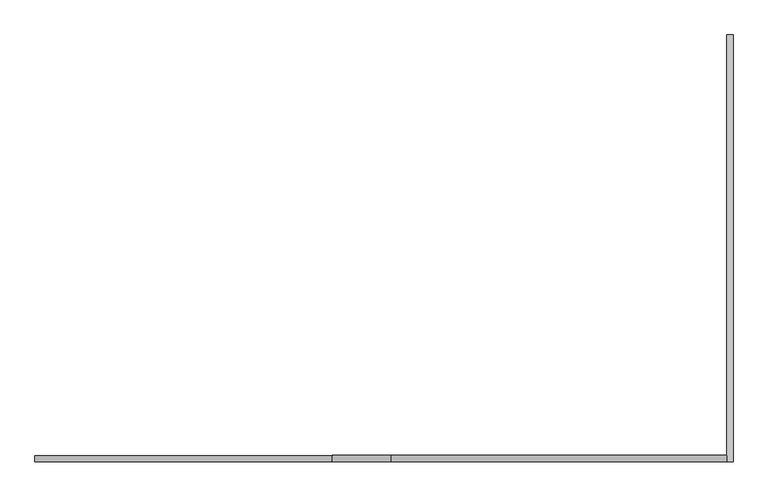
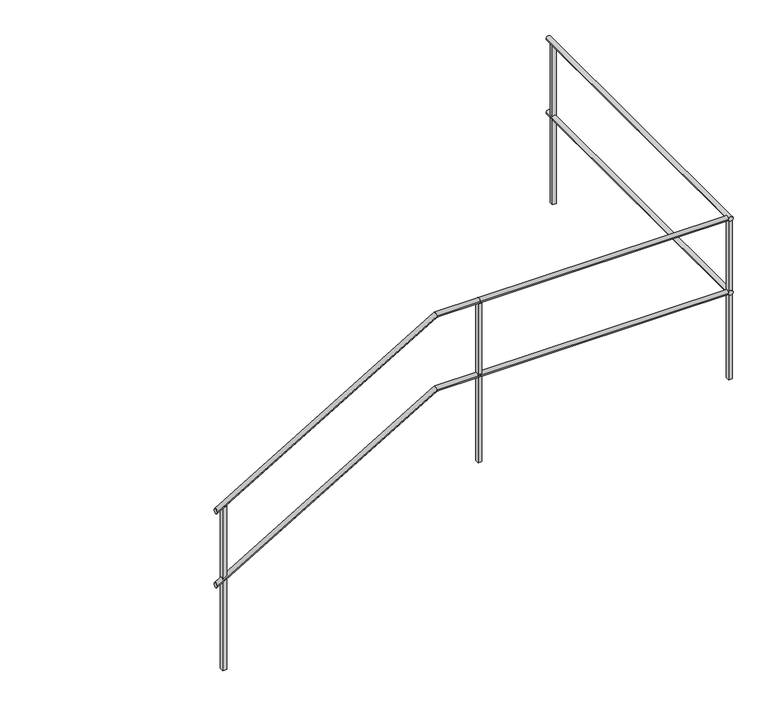
"""IFC4 building model written with IfcOpenShell, lengths in millimetres: railing geometry."""

import ifcopenshell
import ifcopenshell.guid

model = None  # the IFC model being written
_history = None  # IfcOwnerHistory: only IFC2X3 demands one
_inside = {}  # id of a spatial element -> (the spatial element, [elements in it])
_under = {}  # id of a project, library or spatial element -> (it, [spatial elements below it])
_declared = {}  # id of a project -> (the project, [libraries it declares])
_typed = {}  # id of a type object -> (the type object, [elements of that type])
_made_of = {}  # id of a material, layer set ... -> (it, [elements and type objects made of it])


def new_model(schema):
    """Start an empty IFC model of exactly this schema.

    Asked for "IFC4X3", IfcOpenShell would pick the latest addendum, in which some entities
    have other attributes; the version numbers below select the first issue.
    IFC2X3 requires an IfcOwnerHistory on every rooted entity: one is made here for all.
    """
    global model, _history
    if schema == "IFC4X3":
        model = ifcopenshell.file(schema_version=(4, 3, 0, 0))
    else:
        model = ifcopenshell.file(schema=schema)
    _inside.clear()
    _under.clear()
    _declared.clear()
    _typed.clear()
    _made_of.clear()
    _history = None
    if model.schema == "IFC2X3":
        org = make("IfcOrganization", Name="unknown")
        user = make(
            "IfcPersonAndOrganization",
            ThePerson=make("IfcPerson", FamilyName="unknown"),
            TheOrganization=org,
        )
        app = make(
            "IfcApplication",
            ApplicationDeveloper=org,
            Version="unknown",
            ApplicationFullName="unknown",
            ApplicationIdentifier="unknown",
        )
        _history = make(
            "IfcOwnerHistory",
            OwningUser=user,
            OwningApplication=app,
            ChangeAction="ADDED",
            CreationDate=0,
        )
    return model


def make(cls, **values):
    """One entity of the class cls with the attributes given. An attribute that is None is left unset."""
    return model.create_entity(
        cls, **{name: value for name, value in values.items() if value is not None}
    )


def rooted(cls, **values):
    """An entity with a GlobalId (a new one), such as an element, a storey or a relation."""
    return make(cls, GlobalId=ifcopenshell.guid.new(), OwnerHistory=_history, **values)


def si_unit(unit_type, name, prefix=None):
    """IfcSIUnit, for example si_unit("LENGTHUNIT", "METRE", prefix="MILLI")."""
    return make("IfcSIUnit", UnitType=unit_type, Prefix=prefix, Name=name)


def assignment(units):
    """IfcUnitAssignment: the units of a project."""
    return None if units is None else make("IfcUnitAssignment", Units=units)


def point(xyz):
    """IfcCartesianPoint."""
    return None if xyz is None else make("IfcCartesianPoint", Coordinates=xyz)


def direction(xyz):
    """IfcDirection."""
    return None if xyz is None else make("IfcDirection", DirectionRatios=xyz)


def frame(location, z_axis=None, x_axis=None):
    """IfcAxis2Placement3D, a coordinate frame: its origin and axes. An axis left out is left unset."""
    return make(
        "IfcAxis2Placement3D",
        Location=point(location),
        Axis=direction(z_axis),
        RefDirection=direction(x_axis),
    )


def origin():
    """The frame at (0, 0, 0) with its axes left unset."""
    return frame((0.0, 0.0, 0.0))


def place(relative_to, where):
    """IfcLocalPlacement: puts the frame where relative to a parent placement (None: the world)."""
    return make(
        "IfcLocalPlacement", PlacementRelTo=relative_to, RelativePlacement=where
    )


def context(
    kind, dimensions, precision=None, world=None, true_north=None, identifier=None
):
    """IfcGeometricRepresentationContext, for example the 3D "Model" context."""
    return make(
        "IfcGeometricRepresentationContext",
        ContextIdentifier=identifier,
        ContextType=kind,
        CoordinateSpaceDimension=dimensions,
        Precision=precision,
        WorldCoordinateSystem=world,
        TrueNorth=true_north,
    )


def project(units=None, contexts=None):
    """IfcProject with its units and contexts."""
    return rooted(
        "IfcProject",
        Name="project",
        RepresentationContexts=contexts,
        UnitsInContext=assignment(units),
    )


def spatial(cls, under=None, at=None, **own):
    """A site, building, storey or space (cls), placed at a placement, below another one or the project."""
    s = rooted(cls, ObjectPlacement=at, **own)
    if under is not None:
        _under.setdefault(under.id(), (under, []))[1].append(s)
    return s


def polyline(points):
    """IfcPolyline through the points."""
    return make("IfcPolyline", Points=[point(p) for p in points])


def circle_curve(where, radius):
    """IfcCircle in the frame where."""
    return make("IfcCircle", Position=where, Radius=radius)


def ellipse_curve(where, semi_axis1, semi_axis2):
    """IfcEllipse in the frame where."""
    return make(
        "IfcEllipse", Position=where, SemiAxis1=semi_axis1, SemiAxis2=semi_axis2
    )


def outline(outer, holes=None, kind="AREA"):
    """IfcArbitraryClosedProfileDef: a profile drawn as a closed curve; with holes, ...WithVoids."""
    if holes is None:
        return make("IfcArbitraryClosedProfileDef", ProfileType=kind, OuterCurve=outer)
    return make(
        "IfcArbitraryProfileDefWithVoids",
        ProfileType=kind,
        OuterCurve=outer,
        InnerCurves=holes,
    )


def extrude(swept, where, along, depth):
    """IfcExtrudedAreaSolid: the profile swept, set in the frame where, extruded along a direction by depth."""
    return make(
        "IfcExtrudedAreaSolid",
        SweptArea=swept,
        Position=where,
        ExtrudedDirection=direction(along),
        Depth=depth,
    )


def shape(context_of_items, identifier, shape_type, items):
    """IfcShapeRepresentation: the items that make up one representation, for example the "Body"."""
    return make(
        "IfcShapeRepresentation",
        ContextOfItems=context_of_items,
        RepresentationIdentifier=identifier,
        RepresentationType=shape_type,
        Items=items,
    )


def source(mapping_origin, context_of_items, identifier, shape_type, items):
    """IfcRepresentationMap: a shape defined once, which mapped items show again and again."""
    return make(
        "IfcRepresentationMap",
        MappingOrigin=mapping_origin,
        MappedRepresentation=shape(context_of_items, identifier, shape_type, items),
    )


def transform(
    local_origin,
    x_axis=None,
    y_axis=None,
    z_axis=None,
    scale=None,
    scale2=None,
    scale3=None,
    uniform=True,
):
    """IfcCartesianTransformationOperator3D, or its non-uniform kind. x_axis, y_axis, z_axis: its Axis1, 2, 3."""
    if uniform:
        return make(
            "IfcCartesianTransformationOperator3D",
            Axis1=direction(x_axis),
            Axis2=direction(y_axis),
            LocalOrigin=point(local_origin),
            Scale=scale,
            Axis3=direction(z_axis),
        )
    return make(
        "IfcCartesianTransformationOperator3DnonUniform",
        Axis1=direction(x_axis),
        Axis2=direction(y_axis),
        LocalOrigin=point(local_origin),
        Scale=scale,
        Axis3=direction(z_axis),
        Scale2=scale2,
        Scale3=scale3,
    )


def mapped(mapping_source, mapping_target):
    """IfcMappedItem: shows the shape of a source again, moved by a transform."""
    return make(
        "IfcMappedItem", MappingSource=mapping_source, MappingTarget=mapping_target
    )


def made_of(thing, what):
    """Note that an element or type object is made of a material, layer set ...; save() writes the relation."""
    if what is not None:
        _made_of.setdefault(what.id(), (what, []))[1].append(thing)
    return thing


def element(
    cls,
    number,
    at=None,
    inside=None,
    cuts=None,
    type_object=None,
    material=None,
    context=None,
    identifier="Body",
    shape_type=None,
    held_by="IfcProductDefinitionShape",
    body=None,
    shapes=None,
    **own,
):
    """One element of the class cls, such as IfcWall. Its Tag is "e" and its number.

    at: its placement. inside: the storey or other place that contains it. cuts: it is an
    opening in that element (IfcRelVoidsElement). A single representation is given by context,
    identifier, shape_type and body (its items); several are given by shapes. held_by: the class
    of the entity that holds the representations. save() writes the other relations.
    """
    e = rooted(cls, Tag="e%d" % number, ObjectPlacement=at, **own)
    if body is not None:
        shapes = [shape(context, identifier, shape_type, body)]
    if shapes is not None:
        e.Representation = make(held_by, Representations=shapes)
    if inside is not None:
        _inside.setdefault(inside.id(), (inside, []))[1].append(e)
    if cuts is not None:
        rooted(
            "IfcRelVoidsElement", RelatingBuildingElement=cuts, RelatedOpeningElement=e
        )
    if type_object is not None:
        _typed.setdefault(type_object.id(), (type_object, []))[1].append(e)
    return made_of(e, material)


def aggregate(whole, parts):
    """IfcRelAggregates: a whole, such as a stair, and the parts it consists of."""
    return rooted("IfcRelAggregates", RelatingObject=whole, RelatedObjects=parts)


def save(model, path):
    """Write the relations noted so far, then the file.

    IfcRelAggregates (storeys below a building ...), IfcRelContainedInSpatialStructure (elements
    in a storey), IfcRelDefinesByType, IfcRelAssociatesMaterial and IfcRelDeclares: one each for
    every whole, place, type object, material and project.
    """
    for whole, parts in _under.values():
        aggregate(whole, parts)
    for where, things in _inside.values():
        rooted(
            "IfcRelContainedInSpatialStructure",
            RelatedElements=things,
            RelatingStructure=where,
        )
    for kind, things in _typed.values():
        rooted("IfcRelDefinesByType", RelatedObjects=things, RelatingType=kind)
    for what, things in _made_of.values():
        rooted("IfcRelAssociatesMaterial", RelatedObjects=things, RelatingMaterial=what)
    for by, libraries in _declared.values():
        rooted("IfcRelDeclares", RelatingContext=by, RelatedDefinitions=libraries)
    model.write(path)


def plane_surface(at):
    """IfcPlane: the flat surface through the origin of the frame at, square to its z axis."""
    return make("IfcPlane", Position=at)


def cylinder_surface(at, radius):
    """IfcCylindricalSurface: all points at the distance radius from the z axis of the frame at."""
    return make("IfcCylindricalSurface", Position=at, Radius=radius)


def advanced_brep(points, edges, surfaces, faces):
    """IfcAdvancedBrep: a solid bounded by faces that lie on surfaces and meet in shared edges.

    An edge is (start, end): straight between two places in points (the first is 0);
    or (start, end, curve); or (start, end, curve, False) where it runs against its curve.
    A face is (place in surfaces, loops), or (place, loops, False) where it looks against
    its surface's normal. A loop lists edges by number (the first is 1), with a minus sign
    where the edge is run from its end to its start. The first loop is the outer one.
    """
    corners = [point(p) for p in points]
    vertices = [make("IfcVertexPoint", VertexGeometry=c) for c in corners]
    made = []
    for start, end, *more in edges:
        made.append(
            make(
                "IfcEdgeCurve",
                EdgeStart=vertices[start],
                EdgeEnd=vertices[end],
                EdgeGeometry=more[0] if more else make("IfcPolyline", Points=[corners[start], corners[end]]),
                SameSense=more[1] if len(more) > 1 else True,
            )
        )
    hull = []
    for where, loops, *sense in faces:
        bounds = []
        for j, loop in enumerate(loops):
            ring = [make("IfcOrientedEdge", EdgeElement=made[abs(k) - 1], Orientation=k > 0) for k in loop]
            bounds.append(
                make(
                    "IfcFaceOuterBound" if j == 0 else "IfcFaceBound",
                    Bound=make("IfcEdgeLoop", EdgeList=ring),
                    Orientation=True,
                )
            )
        hull.append(make("IfcAdvancedFace", Bounds=bounds, FaceSurface=surfaces[where], SameSense=sense[0] if sense else True))
    return make("IfcAdvancedBrep", Outer=make("IfcClosedShell", CfsFaces=hull))


def railing_1e3f9542(model_context):
    return source(origin(), model_context, "Body", "SolidModel", [
        advanced_brep(
        [(35195.0, -1335.0791411, 899.1723166), (35195.0, -1365.0791411, 899.1723166), (36599.1264386, -1335.0791411, 1734.9618634), (36599.1264386, -1365.0791411, 1734.9618634), (36875.0, -1335.0791411, 1734.9618634), (36875.0, -1365.0791411, 1734.9618634)],
        [
            (0, 1, ellipse_curve(frame((35195.0, -1350.0791411, 899.1723166), z_axis=(-1.0, 0.0, 0.0), x_axis=(0.0, 0.0, -1.0)), 17.4562134, 15.0)),
            (1, 0, ellipse_curve(frame((35195.0, -1350.0791411, 899.1723166), z_axis=(-1.0, 0.0, 0.0), x_axis=(0.0, 0.0, -1.0)), 17.4562134, 15.0)),
            (0, 2),
            (2, 3, ellipse_curve(frame((36599.1264386, -1350.0791411, 1734.9618634), z_axis=(-0.9641817474962142, 0.0, -0.2652424509673112), x_axis=(0.2652424509673106, 0.0, -0.9641817474962145)), 15.5572329, 15.0)),
            (3, 1),
            (3, 2, ellipse_curve(frame((36599.1264386, -1350.0791411, 1734.9618634), z_axis=(-0.9641817474962142, 0.0, -0.2652424509673112), x_axis=(0.2652424509673106, 0.0, -0.9641817474962145)), 15.5572329, 15.0)),
            (4, 5, circle_curve(frame((36875.0, -1350.0791411, 1734.9618634), z_axis=(1.0, 0.0, 0.0), x_axis=(0.0, -1.0, 0.0)), 15.0)),
            (5, 4, circle_curve(frame((36875.0, -1350.0791411, 1734.9618634), z_axis=(1.0, 0.0, 0.0), x_axis=(0.0, -1.0, 0.0)), 15.0)),
            (2, 4),
            (5, 3),
        ],
        [
            plane_surface(frame((35195.0, -1350.0791411, 916.62853), z_axis=(-1.0, 0.0, 0.0), x_axis=(0.0, 1.0, 0.0))),
            cylinder_surface(frame((35202.6722579, -1350.0791411, 903.7391368), z_axis=(-0.8592928844097071, 0.0, -0.511483859767682), x_axis=(0.0, -1.0, 0.0)), 15.0),
            plane_surface(frame((36875.0, -1350.0791411, 1749.9618634), z_axis=(1.0, 0.0, 0.0), x_axis=(0.0, 1.0, 0.0))),
            cylinder_surface(frame((36595.0, -1350.0791411, 1734.9618634), z_axis=(-1.0, 0.0, 0.0), x_axis=(0.0, -1.0, 0.0)), 15.0),
        ],
        [
            (0, [[1, 2]]),
            (1, [[-1, 3, 4, 5]]),
            (1, [[-2, -5, 6, -3]]),
            (2, [[7, 8]]),
            (3, [[-4, 9, -8, 10]]),
            (3, [[-6, -10, -7, -9]]),
        ],
    ),
        advanced_brep(
        [(36875.0, -1335.0791411, 1734.9618634), (36875.0, -1365.0791411, 1734.9618634), (38459.6, -1335.0791411, 1734.9618634), (38459.6, -1365.0791411, 1734.9618634)],
        [
            (0, 1, circle_curve(frame((36875.0, -1350.0791411, 1734.9618634), z_axis=(-1.0, 0.0, 0.0), x_axis=(0.0, -1.0, 0.0)), 15.0)),
            (1, 0, circle_curve(frame((36875.0, -1350.0791411, 1734.9618634), z_axis=(-1.0, 0.0, 0.0), x_axis=(0.0, -1.0, 0.0)), 15.0)),
            (2, 3, circle_curve(frame((38459.6, -1350.0791411, 1734.9618634), z_axis=(1.0, 0.0, 0.0), x_axis=(0.0, -1.0, 0.0)), 15.0)),
            (3, 2, circle_curve(frame((38459.6, -1350.0791411, 1734.9618634), z_axis=(1.0, 0.0, 0.0), x_axis=(0.0, -1.0, 0.0)), 15.0)),
            (0, 2),
            (3, 1),
        ],
        [
            plane_surface(frame((36875.0, -1350.0791411, 1749.9618634), z_axis=(-1.0, 0.0, 0.0), x_axis=(0.0, 1.0, 0.0))),
            plane_surface(frame((38459.6, -1350.0791411, 1749.9618634), z_axis=(1.0, 0.0, 0.0), x_axis=(0.0, 1.0, 0.0))),
            cylinder_surface(frame((36875.0, -1350.0791411, 1734.9618634), z_axis=(-1.0, 0.0, 0.0), x_axis=(0.0, -1.0, 0.0)), 15.0),
        ],
        [
            (0, [[1, 2]]),
            (1, [[3, 4]]),
            (2, [[-1, 5, -4, 6]]),
            (2, [[-2, -6, -3, -5]]),
        ],
    ),
        advanced_brep(
        [(38459.6, -1365.0791411, 1734.9618634), (38489.6, -1365.0791411, 1734.9618634), (38459.6, 649.5208589, 1734.9618634), (38489.6, 649.5208589, 1734.9618634)],
        [
            (0, 1, circle_curve(frame((38474.6, -1365.0791411, 1734.9618634), z_axis=(0.0, -1.0, 0.0), x_axis=(1.0, 0.0, 0.0)), 15.0)),
            (1, 0, circle_curve(frame((38474.6, -1365.0791411, 1734.9618634), z_axis=(0.0, -1.0, 0.0), x_axis=(1.0, 0.0, 0.0)), 15.0)),
            (2, 3, circle_curve(frame((38474.6, 649.5208589, 1734.9618634), z_axis=(0.0, 1.0, 0.0), x_axis=(1.0, 0.0, 0.0)), 15.0)),
            (3, 2, circle_curve(frame((38474.6, 649.5208589, 1734.9618634), z_axis=(0.0, 1.0, 0.0), x_axis=(1.0, 0.0, 0.0)), 15.0)),
            (0, 2),
            (3, 1),
        ],
        [
            plane_surface(frame((38474.6, -1365.0791411, 1749.9618634), z_axis=(0.0, -1.0, 0.0), x_axis=(0.0, 0.0, 1.0))),
            plane_surface(frame((38474.6, 649.5208589, 1749.9618634), z_axis=(0.0, 1.0, 0.0), x_axis=(0.0, 0.0, 1.0))),
            cylinder_surface(frame((38474.6, -1365.0791411, 1734.9618634), z_axis=(0.0, -1.0, 0.0), x_axis=(1.0, 0.0, 0.0)), 15.0),
        ],
        [
            (0, [[1, 2]]),
            (1, [[3, 4]]),
            (2, [[-1, 5, -4, 6]]),
            (2, [[-2, -6, -3, -5]]),
        ],
    ),
        advanced_brep(
        [(35195.0, -1335.0791411, 1399.1723166), (35195.0, -1365.0791411, 1399.1723166), (36599.1264386, -1335.0791411, 2234.9618634), (36599.1264386, -1365.0791411, 2234.9618634), (36875.0, -1335.0791411, 2234.9618634), (36875.0, -1365.0791411, 2234.9618634)],
        [
            (0, 1, ellipse_curve(frame((35195.0, -1350.0791411, 1399.1723166), z_axis=(-1.0, 0.0, 0.0), x_axis=(0.0, 0.0, -1.0)), 17.4562134, 15.0)),
            (1, 0, ellipse_curve(frame((35195.0, -1350.0791411, 1399.1723166), z_axis=(-1.0, 0.0, 0.0), x_axis=(0.0, 0.0, -1.0)), 17.4562134, 15.0)),
            (0, 2),
            (2, 3, ellipse_curve(frame((36599.1264386, -1350.0791411, 2234.9618634), z_axis=(-0.9641817474962142, 0.0, -0.2652424509673112), x_axis=(0.2652424509673106, 0.0, -0.9641817474962145)), 15.5572329, 15.0)),
            (3, 1),
            (3, 2, ellipse_curve(frame((36599.1264386, -1350.0791411, 2234.9618634), z_axis=(-0.9641817474962142, 0.0, -0.2652424509673112), x_axis=(0.2652424509673106, 0.0, -0.9641817474962145)), 15.5572329, 15.0)),
            (4, 5, circle_curve(frame((36875.0, -1350.0791411, 2234.9618634), z_axis=(1.0, 0.0, 0.0), x_axis=(0.0, -1.0, 0.0)), 15.0)),
            (5, 4, circle_curve(frame((36875.0, -1350.0791411, 2234.9618634), z_axis=(1.0, 0.0, 0.0), x_axis=(0.0, -1.0, 0.0)), 15.0)),
            (2, 4),
            (5, 3),
        ],
        [
            plane_surface(frame((35195.0, -1350.0791411, 1416.62853), z_axis=(-1.0, 0.0, 0.0), x_axis=(0.0, 1.0, 0.0))),
            cylinder_surface(frame((35202.6722579, -1350.0791411, 1403.7391368), z_axis=(-0.8592928844097071, 0.0, -0.511483859767682), x_axis=(0.0, -1.0, 0.0)), 15.0),
            plane_surface(frame((36875.0, -1350.0791411, 2249.9618634), z_axis=(1.0, 0.0, 0.0), x_axis=(0.0, 1.0, 0.0))),
            cylinder_surface(frame((36595.0, -1350.0791411, 2234.9618634), z_axis=(-1.0, 0.0, 0.0), x_axis=(0.0, -1.0, 0.0)), 15.0),
        ],
        [
            (0, [[1, 2]]),
            (1, [[-1, 3, 4, 5]]),
            (1, [[-2, -5, 6, -3]]),
            (2, [[7, 8]]),
            (3, [[-4, 9, -8, 10]]),
            (3, [[-6, -10, -7, -9]]),
        ],
    ),
        advanced_brep(
        [(36875.0, -1335.0791411, 2234.9618634), (36875.0, -1365.0791411, 2234.9618634), (38459.6, -1335.0791411, 2234.9618634), (38459.6, -1365.0791411, 2234.9618634)],
        [
            (0, 1, circle_curve(frame((36875.0, -1350.0791411, 2234.9618634), z_axis=(-1.0, 0.0, 0.0), x_axis=(0.0, -1.0, 0.0)), 15.0)),
            (1, 0, circle_curve(frame((36875.0, -1350.0791411, 2234.9618634), z_axis=(-1.0, 0.0, 0.0), x_axis=(0.0, -1.0, 0.0)), 15.0)),
            (2, 3, circle_curve(frame((38459.6, -1350.0791411, 2234.9618634), z_axis=(1.0, 0.0, 0.0), x_axis=(0.0, -1.0, 0.0)), 15.0)),
            (3, 2, circle_curve(frame((38459.6, -1350.0791411, 2234.9618634), z_axis=(1.0, 0.0, 0.0), x_axis=(0.0, -1.0, 0.0)), 15.0)),
            (0, 2),
            (3, 1),
        ],
        [
            plane_surface(frame((36875.0, -1350.0791411, 2249.9618634), z_axis=(-1.0, 0.0, 0.0), x_axis=(0.0, 1.0, 0.0))),
            plane_surface(frame((38459.6, -1350.0791411, 2249.9618634), z_axis=(1.0, 0.0, 0.0), x_axis=(0.0, 1.0, 0.0))),
            cylinder_surface(frame((36875.0, -1350.0791411, 2234.9618634), z_axis=(-1.0, 0.0, 0.0), x_axis=(0.0, -1.0, 0.0)), 15.0),
        ],
        [
            (0, [[1, 2]]),
            (1, [[3, 4]]),
            (2, [[-1, 5, -4, 6]]),
            (2, [[-2, -6, -3, -5]]),
        ],
    ),
        advanced_brep(
        [(38459.6, -1365.0791411, 2234.9618634), (38489.6, -1365.0791411, 2234.9618634), (38459.6, 649.5208589, 2234.9618634), (38489.6, 649.5208589, 2234.9618634)],
        [
            (0, 1, circle_curve(frame((38474.6, -1365.0791411, 2234.9618634), z_axis=(0.0, -1.0, 0.0), x_axis=(1.0, 0.0, 0.0)), 15.0)),
            (1, 0, circle_curve(frame((38474.6, -1365.0791411, 2234.9618634), z_axis=(0.0, -1.0, 0.0), x_axis=(1.0, 0.0, 0.0)), 15.0)),
            (2, 3, circle_curve(frame((38474.6, 649.5208589, 2234.9618634), z_axis=(0.0, 1.0, 0.0), x_axis=(1.0, 0.0, 0.0)), 15.0)),
            (3, 2, circle_curve(frame((38474.6, 649.5208589, 2234.9618634), z_axis=(0.0, 1.0, 0.0), x_axis=(1.0, 0.0, 0.0)), 15.0)),
            (0, 2),
            (3, 1),
        ],
        [
            plane_surface(frame((38474.6, -1365.0791411, 2249.9618634), z_axis=(0.0, -1.0, 0.0), x_axis=(0.0, 0.0, 1.0))),
            plane_surface(frame((38474.6, 649.5208589, 2249.9618634), z_axis=(0.0, 1.0, 0.0), x_axis=(0.0, 0.0, 1.0))),
            cylinder_surface(frame((38474.6, -1365.0791411, 2234.9618634), z_axis=(0.0, -1.0, 0.0), x_axis=(1.0, 0.0, 0.0)), 15.0),
        ],
        [
            (0, [[1, 2]]),
            (1, [[3, 4]]),
            (2, [[-1, 5, -4, 6]]),
            (2, [[-2, -6, -3, -5]]),
        ],
    ),
        extrude(outline(polyline([(38462.1, -1362.5791411), (38462.1, -1337.5791411), (38487.1, -1337.5791411), (38487.1, -1362.5791411), (38462.1, -1362.5791411)])), frame((0.0, 0.0, 1149.9618634), z_axis=(0.0, 0.0, 1.0), x_axis=(1.0, 0.0, 0.0)), (0.0, 0.0, 1.0), 1070.0),
        extrude(outline(polyline([(36862.5, -1362.5791411), (36862.5, -1337.5791411), (36887.5, -1337.5791411), (36887.5, -1362.5791411), (36862.5, -1362.5791411)])), frame((0.0, 0.0, 1149.9618634), z_axis=(0.0, 0.0, 1.0), x_axis=(1.0, 0.0, 0.0)), (0.0, 0.0, 1.0), 1070.0),
        extrude(outline(polyline([(38487.1, 587.0208589), (38462.1, 587.0208589), (38462.1, 612.0208589), (38487.1, 612.0208589), (38487.1, 587.0208589)])), frame((0.0, 0.0, 1149.9618634), z_axis=(0.0, 0.0, 1.0), x_axis=(1.0, 0.0, 0.0)), (0.0, 0.0, 1.0), 1070.0),
        extrude(outline(polyline([(1408.9499586, 35232.5), (316.62853, 35232.5), (316.62853, 35257.5), (1423.830911, 35257.5), (1408.9499586, 35232.5)])), frame((0.0, -1362.5791411, 0.0), z_axis=(0.0, 1.0, 0.0), x_axis=(0.0, 0.0, 1.0)), (0.0, 0.0, 1.0), 25.0),
    ])


if __name__ == "__main__":
    model = new_model("IFC4")
    model_context = context("Model", 3, world=origin())
    ifc_project = project(units=[si_unit("LENGTHUNIT", "METRE", prefix="MILLI")], contexts=[model_context])
    site = spatial("IfcSite", under=ifc_project)
    building = spatial("IfcBuilding", under=site)
    placement = place(None, origin())
    railing_shape = railing_1e3f9542(model_context)
    element("IfcRailing", 1, at=placement, inside=building, context=model_context, shape_type="MappedRepresentation", body=[
        mapped(railing_shape, transform((0.0, 0.0, 0.0), x_axis=(1.0, 0.0, 0.0), y_axis=(0.0, 1.0, 0.0), z_axis=(0.0, 0.0, 1.0))),
    ])
    save(model, "model.ifc")
